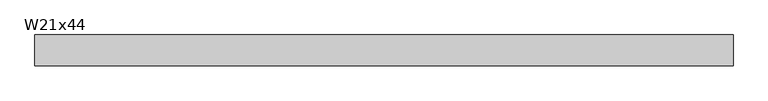
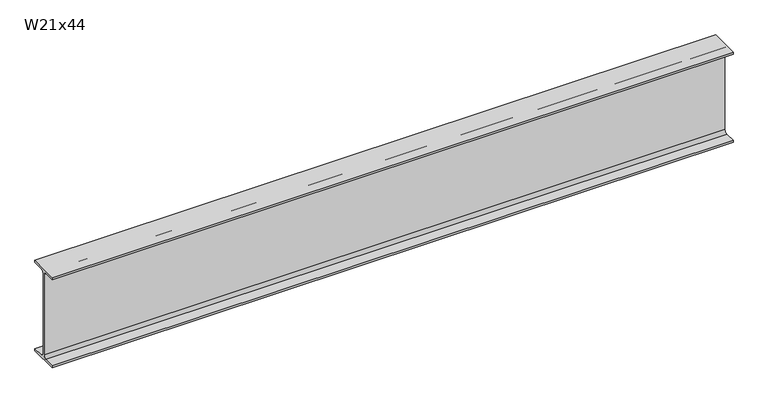
"""IFC4 building model written with IfcOpenShell, lengths in millimetres: beam geometry, RME W-Wide Flange : W21x44."""

from ifc_helpers import new_model, si_unit, point, frame, frame_2d, origin, place, context, project, spatial, polyline, circle_curve, trimmed, segment, composite_curve, outline, extrude, source, transform, mapped, element, save


def w21x44_847699e2(model_context):
    return source(origin(), model_context, "Body", "SweptSolid", [
        extrude(outline(composite_curve([segment(polyline([(82.55, -251.46), (82.55, -262.89), (-82.55, -262.89), (-82.55, -251.46), (-21.59, -251.46)]), True, "CONTINUOUS"), segment(trimmed(circle_curve(frame_2d((-21.59, -234.315)), 17.145), [point((-21.59, -251.46))], [point((-4.445, -234.315))], True, "CARTESIAN"), True, "CONTINUOUS"), segment(polyline([(-4.445, -234.315), (-4.445, 234.315)]), True, "CONTINUOUS"), segment(trimmed(circle_curve(frame_2d((-21.59, 234.315)), 17.145), [point((-4.445, 234.315))], [point((-21.59, 251.46))], True, "CARTESIAN"), True, "CONTINUOUS"), segment(polyline([(-21.59, 251.46), (-82.55, 251.46), (-82.55, 262.89), (82.55, 262.89), (82.55, 251.46), (21.59, 251.46)]), True, "CONTINUOUS"), segment(trimmed(circle_curve(frame_2d((21.59, 234.315)), 17.145), [point((21.59, 251.46))], [point((4.445, 234.315))], True, "CARTESIAN"), True, "CONTINUOUS"), segment(polyline([(4.445, 234.315), (4.445, -234.315)]), True, "CONTINUOUS"), segment(trimmed(circle_curve(frame_2d((21.59, -234.315)), 17.145), [point((4.445, -234.315))], [point((21.59, -251.46))], True, "CARTESIAN"), True, "CONTINUOUS"), segment(polyline([(21.59, -251.46), (82.55, -251.46)]), True, "CONTINUOUS")], self_intersect=False)), frame((-1867.788845, 0.0, 0.0), z_axis=(1.0, 0.0, 0.0), x_axis=(0.0, 1.0, 0.0)), (0.0, 0.0, 1.0), 3753.23069),
    ])


if __name__ == "__main__":
    model = new_model("IFC4")
    model_context = context("Model", 3, world=origin())
    ifc_project = project(units=[si_unit("LENGTHUNIT", "METRE", prefix="MILLI")], contexts=[model_context])
    site = spatial("IfcSite", under=ifc_project)
    building = spatial("IfcBuilding", under=site)
    placement = place(None, origin())
    w21x44_shape = w21x44_847699e2(model_context)
    element("IfcBeam", 1, ObjectType="RME W-Wide Flange : W21x44", at=placement, inside=building, context=model_context, shape_type="MappedRepresentation", body=[
        mapped(w21x44_shape, transform((0.0, 0.0, 0.0), x_axis=(1.0, 0.0, 0.0), y_axis=(0.0, 1.0, 0.0), z_axis=(0.0, 0.0, 1.0))),
    ])
    save(model, "model.ifc")

# Revit data of these elements
# Type "RME W-Wide Flange : W21x44"
#   WELD P [instance default] = ""
#   WELD LE [instance default] = ""
#   WELD D [instance default] = ""
#   TOP SECTION SIZE [instance default] = ""
#   TOP SECTION LENGTH [instance default] = ""
#   REMARKS [instance default] = ""
#   REINF TYPE [instance default] = ""
#   Nominal Size = "W24"
#   End Bearing Capacity [instance default] = ""
#   BOT SECTION SIZE [instance default] = ""
#   BOT SECTION LENGTH [instance default] = ""
#   Assembly Code = "B10"
#   W = 44
#   Start Extension Calculation [instance default] = 10' - 0"
#   Start Extension [instance default] = -0' - 0 1/2"
#   End Extension Calculation [instance default] = 10' - 0"
#   End Extension [instance default] = -0' - 0 1/2"
#   Length [instance default] = 5' - 0"
#   bf = 0' - 6 1/2"
#   d = 1' - 8.7"
#   k = 0' - 1 1/8"
#   k2 = 0' - 0.675"
#   tf = 0' - 0.45"
#   tw = 0' - 0.35"
#   A = 0.0902778 SF
#   Structural Material [instance default] = Metal - Steel - ASTM A992
# Element 1 (IfcBeam, "RME W-Wide Flange : W21x44")
#   Length = 13' - 0"
#   Materials on its faces: "Metal - Steel - ASTM A992"
# Materials
#   "Metal - Steel - ASTM A992": class "Metal", colour RGB 255 128 0, transparency 0
